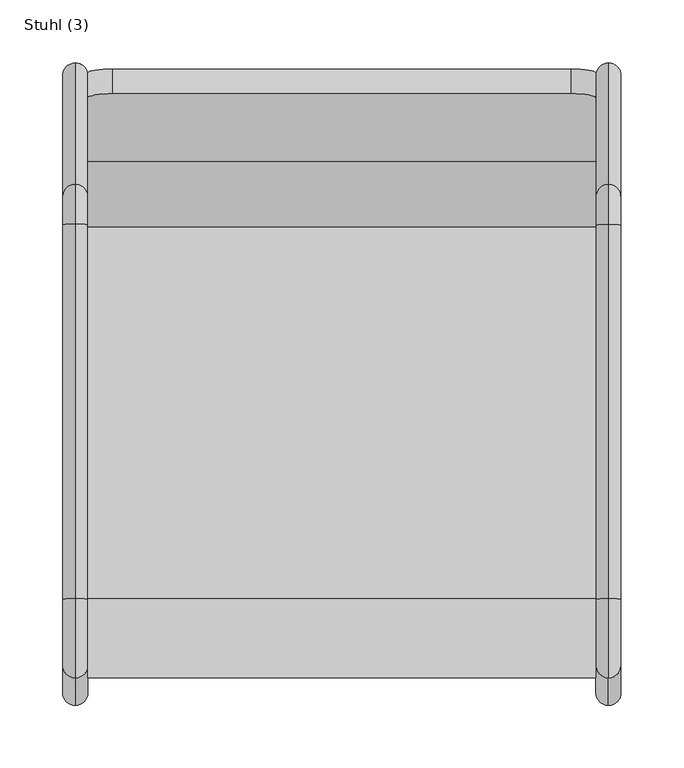
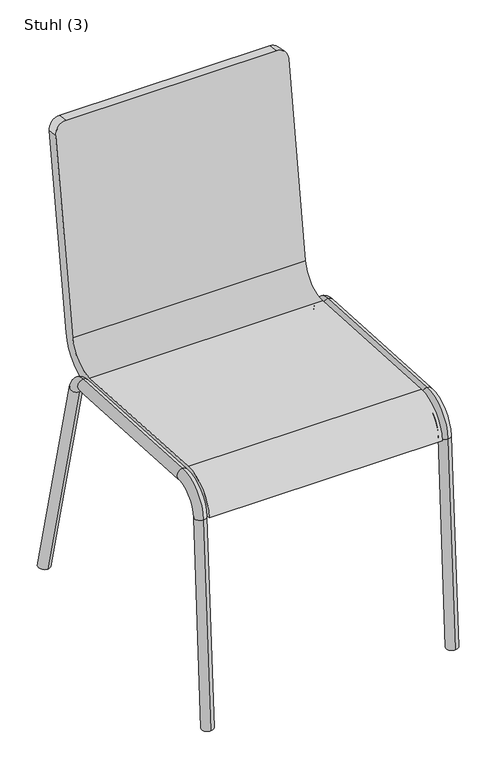
"""IFC4 building model written with IfcOpenShell, lengths in millimetres: furniture geometry, Stuhl (3) : Sessel."""

from ifc_helpers import new_model, si_unit, point, frame, origin, place, context, project, spatial, polyline, circle_curve, ellipse_curve, trimmed, source, transform, mapped, element, save
from ifc_brep_helpers import plane_surface, cylinder_surface, revolved_surface, advanced_brep


def stuhl_3_dbe21b2d(model_context):
    return source(origin(), model_context, "Body", "AdvancedBrep", [
        advanced_brep(
        [(-139.5255992, 4.9530016, 0.0), (-139.5255992, 25.5652742, 0.0), (-129.5255992, -476.7023393, 0.0), (-149.5255992, -476.7023393, 0.0), (-139.5255992, -466.6854234, 0.0), (-139.5255992, -90.5686349, 383.1163586), (-139.5255992, -71.1627204, 387.9547965), (-139.5255992, -104.2517001, 394.4621992), (-139.5255992, -103.0898724, 414.4284246), (-139.5255992, -402.6537429, 411.8261096), (-139.5255992, -401.4919152, 431.792335), (-139.5255992, -444.909849, 374.2173141), (-139.5255992, -464.8760744, 375.3791418), (-139.5255992, -486.685452, 0.5809138)],
        [
            (0, 1, ellipse_curve(frame((-139.5255992, 15.2591379, 0.0), z_axis=(0.0, 0.0, -1.0), x_axis=(0.0, 1.0, 0.0)), 10.3061363, 10.0)),
            (1, 0, ellipse_curve(frame((-139.5255992, 15.2591379, 0.0), z_axis=(0.0, 0.0, -1.0), x_axis=(0.0, 1.0, 0.0)), 10.3061363, 10.0)),
            (2, 3),
            (3, 4, ellipse_curve(frame((-139.5255992, -476.7023393, 0.0), z_axis=(0.0, 0.0, -1.0), x_axis=(0.0, 1.0, 0.0)), 10.0169159, 10.0)),
            (4, 2, ellipse_curve(frame((-139.5255992, -476.7023393, 0.0), z_axis=(0.0, 0.0, -1.0), x_axis=(0.0, 1.0, 0.0)), 10.0169159, 10.0)),
            (5, 6, circle_curve(frame((-139.5255992, -80.8656776, 385.5355776), z_axis=(0.0, 0.24192189559966623, -0.9702957262759968), x_axis=(0.0, 0.9702957262759968, 0.24192189559966623)), 10.0)),
            (6, 1),
            (0, 5),
            (6, 5, circle_curve(frame((-139.5255992, -80.8656776, 385.5355776), z_axis=(0.0, 0.24192189559966623, -0.9702957262759968), x_axis=(0.0, 0.9702957262759968, 0.24192189559966623)), 10.0)),
            (5, 7, circle_curve(frame((-139.5255992, -105.1230708, 379.4875302), z_axis=(1.0, 0.0, 0.0), x_axis=(0.0, 0.9702957262759969, 0.2419218955996659)), 15.0)),
            (7, 8, circle_curve(frame((-139.5255992, -103.6707862, 404.4453119), z_axis=(0.0, 0.998311269703977, -0.058091383027376764), x_axis=(0.0, 0.058091383027376764, 0.998311269703977)), 10.0)),
            (8, 6, circle_curve(frame((-139.5255992, -105.1230708, 379.4875302), z_axis=(-1.0, 0.0, 0.0), x_axis=(0.0, 0.9702957262759969, 0.2419218955996659)), 35.0)),
            (8, 7, circle_curve(frame((-139.5255992, -103.6707862, 404.4453119), z_axis=(0.0, 0.9983112697039765, -0.05809138302738498), x_axis=(0.0, 0.05809138302738498, 0.9983112697039765)), 10.0)),
            (7, 9),
            (9, 10, circle_curve(frame((-139.5255992, -402.0728291, 421.8092223), z_axis=(0.0, 0.9983112697039764, -0.058091383027386895), x_axis=(0.0, 0.058091383027386895, 0.9983112697039764)), 10.0)),
            (10, 8),
            (10, 9, circle_curve(frame((-139.5255992, -402.0728291, 421.8092223), z_axis=(0.0, 0.9983112697039764, -0.058091383027386895), x_axis=(0.0, 0.058091383027386895, 0.9983112697039764)), 10.0)),
            (9, 11, circle_curve(frame((-139.5255992, -404.9773982, 371.8936588), z_axis=(1.0, 0.0, 0.0), x_axis=(0.0, 0.05809138302738633, 0.9983112697039764)), 40.0)),
            (11, 12, circle_curve(frame((-139.5255992, -454.8929617, 374.7982279), z_axis=(0.0, 0.058091383027391474, 0.9983112697039761), x_axis=(0.0, -0.9983112697039761, 0.058091383027391474)), 10.0)),
            (12, 10, circle_curve(frame((-139.5255992, -404.9773982, 371.8936588), z_axis=(-1.0, 0.0, 0.0), x_axis=(0.0, 0.05809138302738633, 0.9983112697039764)), 60.0)),
            (12, 11, circle_curve(frame((-139.5255992, -454.8929617, 374.7982279), z_axis=(0.0, 0.05809138302739081, 0.9983112697039762), x_axis=(0.0, -0.9983112697039762, 0.05809138302739081)), 10.0)),
            (2, 13, circle_curve(frame((-139.5255992, -476.7023393, 0.0), z_axis=(0.0, -0.058091383027392335, -0.9983112697039761), x_axis=(0.0, -0.9983112697039761, 0.058091383027392335)), 10.0)),
            (13, 3, circle_curve(frame((-139.5255992, -476.7023393, 0.0), z_axis=(0.0, -0.058091383027392335, -0.9983112697039761), x_axis=(0.0, -0.9983112697039761, 0.058091383027392335)), 10.0)),
            (11, 4),
            (13, 12),
        ],
        [
            plane_surface(frame((-102.1053, 50.7055201, 0.0), z_axis=(0.0, 0.0, -1.0), x_axis=(-1.0, 0.0, 0.0))),
            cylinder_surface(frame((-139.5255992, 17.8692882, -10.4687411), z_axis=(0.0, 0.24192189559966623, -0.9702957262759968), x_axis=(0.0, 0.9702957262759968, 0.24192189559966623)), 10.0),
            revolved_surface(trimmed(ellipse_curve(frame((-139.5255992, -80.8656776, 385.5355776), z_axis=(0.0, 0.2419218955996659, -0.9702957262759969), x_axis=(0.0, 0.9702957262759969, 0.2419218955996659)), 10.0, 10.0), [point((-139.5255992, -90.5686349, 383.1163586))], [point((-139.5255992, -71.1627204, 387.9547965))], True, "CARTESIAN"), (-159.5255992, -105.1230708, 379.4875302), (1.0, 0.0, 0.0)),
            revolved_surface(trimmed(ellipse_curve(frame((-139.5255992, -80.8656776, 385.5355776), z_axis=(0.0, 0.2419218955996659, -0.9702957262759969), x_axis=(0.0, 0.9702957262759969, 0.2419218955996659)), 10.0, 10.0), [point((-139.5255992, -71.1627204, 387.9547965))], [point((-139.5255992, -90.5686349, 383.1163586))], True, "CARTESIAN"), (-159.5255992, -105.1230708, 379.4875302), (1.0, 0.0, 0.0)),
            cylinder_surface(frame((-139.5255992, -103.6707862, 404.4453119), z_axis=(0.0, 0.9983112697039764, -0.058091383027386895), x_axis=(0.0, 0.058091383027386895, 0.9983112697039764)), 10.0),
            revolved_surface(trimmed(ellipse_curve(frame((-139.5255992, -402.0728291, 421.8092223), z_axis=(0.0, 0.9983112697039764, -0.05809138302738631), x_axis=(0.0, 0.05809138302738631, 0.9983112697039764)), 10.0, 10.0), [point((-139.5255992, -402.6537429, 411.8261096))], [point((-139.5255992, -401.4919152, 431.792335))], True, "CARTESIAN"), (-159.5255992, -404.9773982, 371.8936588), (1.0, 0.0, 0.0)),
            revolved_surface(trimmed(ellipse_curve(frame((-139.5255992, -402.0728291, 421.8092223), z_axis=(0.0, 0.9983112697039764, -0.05809138302738631), x_axis=(0.0, 0.05809138302738631, 0.9983112697039764)), 10.0, 10.0), [point((-139.5255992, -401.4919152, 431.792335))], [point((-139.5255992, -402.6537429, 411.8261096))], True, "CARTESIAN"), (-159.5255992, -404.9773982, 371.8936588), (1.0, 0.0, 0.0)),
            plane_surface(frame((-159.5255992, -476.7023393, 0.0), z_axis=(0.0, -0.058091383027392335, -0.9983112697039761), x_axis=(1.0, 0.0, 0.0))),
            cylinder_surface(frame((-139.5255992, -454.8929617, 374.7982279), z_axis=(0.0, 0.058091383027392335, 0.9983112697039761), x_axis=(0.0, -0.9983112697039761, 0.058091383027392335)), 10.0),
        ],
        [
            (0, [[1, 2]]),
            (0, [[3, 4, 5]]),
            (1, [[6, 7, -1, 8]]),
            (1, [[9, -8, -2, -7]]),
            (2, [[-6, 10, 11, 12]]),
            (3, [[-9, -12, 13, -10]]),
            (4, [[-11, 14, 15, 16]]),
            (4, [[-13, -16, 17, -14]]),
            (5, [[-15, 18, 19, 20]]),
            (6, [[-17, -20, 21, -18]]),
            (7, [[22, 23, -3]]),
            (8, [[-19, 24, -4, -23, 25]]),
            (8, [[-21, -25, -22, -5, -24]]),
        ],
    ),
        advanced_brep(
        [(-554.6850007, -476.7023393, 0.0), (-564.6850007, -486.685452, 0.5809138), (-574.6850007, -476.7023393, 0.0), (-564.6850007, -90.5686349, 383.1163586), (-564.6850007, -71.1627204, 387.9547965), (-564.6850007, 25.5652742, 0.0), (-564.6850007, 4.9530016, 0.0), (-564.6850007, -466.6854234, 0.0), (-564.6850007, -103.0898724, 414.4284246), (-564.6850007, -104.2517001, 394.4621992), (-564.6850007, -402.6537429, 411.8261096), (-564.6850007, -401.4919152, 431.792335), (-564.6850007, -444.909849, 374.2173141), (-564.6850007, -464.8760744, 375.3791418)],
        [
            (0, 1, circle_curve(frame((-564.6850007, -476.7023393, 0.0), z_axis=(0.0, -0.058091383027392335, -0.9983112697039761), x_axis=(0.0, -0.9983112697039761, 0.058091383027392335)), 10.0)),
            (1, 2, circle_curve(frame((-564.6850007, -476.7023393, 0.0), z_axis=(0.0, -0.058091383027392335, -0.9983112697039761), x_axis=(0.0, -0.9983112697039761, 0.058091383027392335)), 10.0)),
            (2, 0),
            (3, 4, circle_curve(frame((-564.6850007, -80.8656776, 385.5355776), z_axis=(0.0, 0.24192189559966623, -0.9702957262759968), x_axis=(0.0, 0.9702957262759968, 0.24192189559966623)), 10.0)),
            (4, 5),
            (5, 6, ellipse_curve(frame((-564.6850007, 15.2591379, 0.0), z_axis=(0.0, 0.0, 1.0), x_axis=(0.0, 1.0, 0.0)), 10.3061363, 10.0)),
            (6, 3),
            (4, 3, circle_curve(frame((-564.6850007, -80.8656776, 385.5355776), z_axis=(0.0, 0.24192189559966623, -0.9702957262759968), x_axis=(0.0, 0.9702957262759968, 0.24192189559966623)), 10.0)),
            (6, 5, ellipse_curve(frame((-564.6850007, 15.2591379, 0.0), z_axis=(0.0, 0.0, 1.0), x_axis=(0.0, 1.0, 0.0)), 10.3061363, 10.0)),
            (2, 7, ellipse_curve(frame((-564.6850007, -476.7023393, 0.0), z_axis=(0.0, 0.0, -1.0), x_axis=(0.0, 1.0, 0.0)), 10.0169159, 10.0)),
            (7, 0, ellipse_curve(frame((-564.6850007, -476.7023393, 0.0), z_axis=(0.0, 0.0, -1.0), x_axis=(0.0, 1.0, 0.0)), 10.0169159, 10.0)),
            (8, 9, circle_curve(frame((-564.6850007, -103.6707862, 404.4453119), z_axis=(0.0, -0.9983112697039764, 0.058091383027386895), x_axis=(0.0, 0.058091383027386895, 0.9983112697039764)), 10.0)),
            (9, 10),
            (10, 11, circle_curve(frame((-564.6850007, -402.0728291, 421.8092223), z_axis=(0.0, 0.9983112697039764, -0.058091383027386895), x_axis=(0.0, 0.058091383027386895, 0.9983112697039764)), 10.0)),
            (11, 8),
            (9, 8, circle_curve(frame((-564.6850007, -103.6707862, 404.4453119), z_axis=(0.0, -0.9983112697039764, 0.058091383027386895), x_axis=(0.0, 0.058091383027386895, 0.9983112697039764)), 10.0)),
            (11, 10, circle_curve(frame((-564.6850007, -402.0728291, 421.8092223), z_axis=(0.0, 0.9983112697039764, -0.058091383027386895), x_axis=(0.0, 0.058091383027386895, 0.9983112697039764)), 10.0)),
            (10, 12, circle_curve(frame((-564.6850007, -404.9773982, 371.8936588), z_axis=(1.0, 0.0, 0.0), x_axis=(0.0, 0.05809138302738633, 0.9983112697039764)), 40.0)),
            (12, 13, circle_curve(frame((-564.6850007, -454.8929617, 374.7982279), z_axis=(0.0, 0.058091383027391474, 0.9983112697039761), x_axis=(0.0, -0.9983112697039761, 0.058091383027391474)), 10.0)),
            (13, 11, circle_curve(frame((-564.6850007, -404.9773982, 371.8936588), z_axis=(-1.0, 0.0, 0.0), x_axis=(0.0, 0.05809138302738633, 0.9983112697039764)), 60.0)),
            (13, 12, circle_curve(frame((-564.6850007, -454.8929617, 374.7982279), z_axis=(0.0, 0.05809138302739081, 0.9983112697039762), x_axis=(0.0, -0.9983112697039762, 0.05809138302739081)), 10.0)),
            (12, 7),
            (1, 13),
            (3, 9, circle_curve(frame((-564.6850007, -105.1230708, 379.4875302), z_axis=(1.0, 0.0, 0.0), x_axis=(0.0, 0.9702957262759969, 0.2419218955996659)), 15.0)),
            (8, 4, circle_curve(frame((-564.6850007, -105.1230708, 379.4875302), z_axis=(-1.0, 0.0, 0.0), x_axis=(0.0, 0.9702957262759969, 0.2419218955996659)), 35.0)),
        ],
        [
            plane_surface(frame((-544.6850007, -476.7023393, 0.0), z_axis=(0.0, -0.058091383027392335, -0.9983112697039761), x_axis=(-1.0, 0.0, 0.0))),
            cylinder_surface(frame((-564.6850007, 17.8692882, -10.4687411), z_axis=(0.0, 0.24192189559966623, -0.9702957262759968), x_axis=(0.0, 0.9702957262759968, 0.24192189559966623)), 10.0),
            plane_surface(frame((-102.1053, 50.7055201, 0.0), z_axis=(0.0, 0.0, -1.0), x_axis=(-1.0, 0.0, 0.0))),
            cylinder_surface(frame((-564.6850007, -103.6707862, 404.4453119), z_axis=(0.0, 0.9983112697039764, -0.058091383027386895), x_axis=(0.0, 0.058091383027386895, 0.9983112697039764)), 10.0),
            revolved_surface(trimmed(ellipse_curve(frame((-564.6850007, -402.0728291, 421.8092223), z_axis=(0.0, 0.9983112697039764, -0.05809138302738631), x_axis=(0.0, 0.05809138302738631, 0.9983112697039764)), 10.0, 10.0), [point((-564.6850007, -402.6537429, 411.8261096))], [point((-564.6850007, -401.4919152, 431.792335))], True, "CARTESIAN"), (-544.6850007, -404.9773982, 371.8936588), (1.0, 0.0, 0.0)),
            revolved_surface(trimmed(ellipse_curve(frame((-564.6850007, -402.0728291, 421.8092223), z_axis=(0.0, 0.9983112697039764, -0.05809138302738631), x_axis=(0.0, 0.05809138302738631, 0.9983112697039764)), 10.0, 10.0), [point((-564.6850007, -401.4919152, 431.792335))], [point((-564.6850007, -402.6537429, 411.8261096))], True, "CARTESIAN"), (-544.6850007, -404.9773982, 371.8936588), (1.0, 0.0, 0.0)),
            cylinder_surface(frame((-564.6850007, -454.8929617, 374.7982279), z_axis=(0.0, 0.058091383027392335, 0.9983112697039761), x_axis=(0.0, -0.9983112697039761, 0.058091383027392335)), 10.0),
            revolved_surface(trimmed(ellipse_curve(frame((-564.6850007, -80.8656776, 385.5355776), z_axis=(0.0, 0.2419218955996659, -0.9702957262759969), x_axis=(0.0, 0.9702957262759969, 0.2419218955996659)), 10.0, 10.0), [point((-564.6850007, -90.5686349, 383.1163586))], [point((-564.6850007, -71.1627204, 387.9547965))], True, "CARTESIAN"), (-544.6850007, -105.1230708, 379.4875302), (1.0, 0.0, 0.0)),
            revolved_surface(trimmed(ellipse_curve(frame((-564.6850007, -80.8656776, 385.5355776), z_axis=(0.0, 0.2419218955996659, -0.9702957262759969), x_axis=(0.0, 0.9702957262759969, 0.2419218955996659)), 10.0, 10.0), [point((-564.6850007, -71.1627204, 387.9547965))], [point((-564.6850007, -90.5686349, 383.1163586))], True, "CARTESIAN"), (-544.6850007, -105.1230708, 379.4875302), (1.0, 0.0, 0.0)),
        ],
        [
            (0, [[1, 2, 3]]),
            (1, [[4, 5, 6, 7]]),
            (1, [[8, -7, 9, -5]]),
            (2, [[-3, 10, 11]]),
            (2, [[-6, -9]]),
            (3, [[12, 13, 14, 15]]),
            (3, [[16, -15, 17, -13]]),
            (4, [[-14, 18, 19, 20]]),
            (5, [[-17, -20, 21, -18]]),
            (6, [[-19, 22, -10, -2, 23]]),
            (6, [[-21, -23, -1, -11, -22]]),
            (7, [[-4, 24, -12, 25]]),
            (8, [[-8, -25, -16, -24]]),
        ],
    ),
        advanced_brep(
        [(-149.6053, -105.450673, 414.5657988), (-149.6053, -401.4919152, 431.792335), (-149.6053, -464.8760744, 375.3791418), (-149.6053, -444.909849, 374.2173141), (-149.6053, -402.6537429, 411.8261096), (-149.6053, -106.6125007, 394.5995734), (-149.6053, -33.3149934, 454.1347035), (-149.6053, 17.5412109, 794.4215124), (-149.6053, -2.2391064, 797.3777006), (-149.6053, -53.0953107, 457.0908917), (-554.6053, -105.450673, 414.5657988), (-554.6053, -53.0953107, 457.0908917), (-554.6053, -2.2391064, 797.3777006), (-554.6053, 17.5412109, 794.4215124), (-554.6053, -33.3149934, 454.1347035), (-554.6053, -106.6125007, 394.5995734), (-554.6053, -402.6537429, 411.8261096), (-554.6053, -444.909849, 374.2173141), (-554.6053, -464.8760744, 375.3791418), (-554.6053, -401.4919152, 431.792335), (-534.6053, 20.4973991, 814.2018297), (-169.6053, 20.4973991, 814.2018297), (-534.6053, 0.7170819, 817.1580179), (-169.6053, 0.7170819, 817.1580179)],
        [
            (0, 1),
            (1, 2, circle_curve(frame((-149.6053, -404.9773982, 371.8936588), z_axis=(1.0, 0.0, 0.0), x_axis=(0.0, 1.0, 0.0)), 60.0)),
            (2, 3),
            (3, 4, circle_curve(frame((-149.6053, -404.9773982, 371.8936588), z_axis=(-1.0, 0.0, 0.0), x_axis=(0.0, 1.0, 0.0)), 40.0)),
            (4, 5),
            (5, 6, circle_curve(frame((-149.6053, -102.5461039, 464.4813623), z_axis=(1.0, 0.0, 0.0), x_axis=(0.0, 1.0, 0.0)), 70.0)),
            (6, 7),
            (7, 8),
            (8, 9),
            (9, 0, circle_curve(frame((-149.6053, -102.5461039, 464.4813623), z_axis=(-1.0, 0.0, 0.0), x_axis=(0.0, 1.0, 0.0)), 50.0)),
            (10, 11, circle_curve(frame((-554.6053, -102.5461039, 464.4813623), z_axis=(1.0, 0.0, 0.0), x_axis=(0.0, 1.0, 0.0)), 50.0)),
            (11, 12),
            (12, 13),
            (13, 14),
            (14, 15, circle_curve(frame((-554.6053, -102.5461039, 464.4813623), z_axis=(-1.0, 0.0, 0.0), x_axis=(0.0, 1.0, 0.0)), 70.0)),
            (15, 16),
            (16, 17, circle_curve(frame((-554.6053, -404.9773982, 371.8936588), z_axis=(1.0, 0.0, 0.0), x_axis=(0.0, 1.0, 0.0)), 40.0)),
            (17, 18),
            (18, 19, circle_curve(frame((-554.6053, -404.9773982, 371.8936588), z_axis=(-1.0, 0.0, 0.0), x_axis=(0.0, 1.0, 0.0)), 60.0)),
            (19, 10),
            (0, 10),
            (19, 1),
            (18, 2),
            (17, 3),
            (16, 4),
            (15, 5),
            (14, 6),
            (13, 20, circle_curve(frame((-534.6053, 17.5412109, 794.4215124), z_axis=(0.0, 0.9890158633619166, -0.14780941112961252), x_axis=(1.0, 0.0, 0.0)), 20.0)),
            (20, 21),
            (21, 7, circle_curve(frame((-169.6053, 17.5412109, 794.4215124), z_axis=(0.0, 0.9890158633619166, -0.14780941112961252), x_axis=(-1.0, 0.0, 0.0)), 20.0)),
            (20, 22),
            (22, 23),
            (23, 21),
            (11, 9),
            (8, 23, circle_curve(frame((-169.6053, -2.2391064, 797.3777006), z_axis=(0.0, -0.9890158633619166, 0.14780941112961252), x_axis=(-1.0, 0.0, 0.0)), 20.0)),
            (22, 12, circle_curve(frame((-534.6053, -2.2391064, 797.3777006), z_axis=(0.0, -0.9890158633619166, 0.14780941112961252), x_axis=(1.0, 0.0, 0.0)), 20.0)),
        ],
        [
            plane_surface(frame((-149.6053, -399.2468499, 431.6616954), z_axis=(1.0000000000000002, 0.0, 0.0), x_axis=(0.0, -0.9983112697039764, 0.05809138302738736))),
            plane_surface(frame((-554.6053, -399.2468499, 431.6616954), z_axis=(-1.0000000000000002, 0.0, 0.0), x_axis=(0.0, 0.9983112697039764, -0.05809138302738736))),
            plane_surface(frame((-149.6053, -105.450673, 414.5657988), z_axis=(0.0, 0.05809138302738736, 0.9983112697039764), x_axis=(-1.0, 0.0, 0.0))),
            cylinder_surface(frame((-554.6053, -404.9773982, 371.8936588), z_axis=(1.0, 0.0, 0.0), x_axis=(0.0, 1.0, 0.0)), 60.0),
            plane_surface(frame((-149.6053, -464.8760744, 375.3791418), z_axis=(0.0, -0.058091383027390926, -0.9983112697039762), x_axis=(-1.0, 0.0, 0.0))),
            revolved_surface(polyline([(-554.6053, -364.9773982, 371.8936588), (-149.6053, -364.9773982, 371.8936588)]), (-554.6053, -404.9773982, 371.8936588), (-1.0, 0.0, 0.0)),
            plane_surface(frame((-149.6053, -402.6537429, 411.8261096), z_axis=(0.0, -0.05809138302738756, -0.9983112697039763), x_axis=(-1.0, 0.0, 0.0))),
            cylinder_surface(frame((-554.6053, -102.5461039, 464.4813623), z_axis=(1.0, 0.0, 0.0), x_axis=(0.0, 1.0, 0.0)), 70.0),
            plane_surface(frame((-149.6053, -33.3149934, 454.1347035), z_axis=(0.0, 0.9890158633619166, -0.1478094111296125), x_axis=(-1.0, 0.0, 0.0))),
            plane_surface(frame((-149.6053, 20.4973991, 814.2018297), z_axis=(0.0, 0.14780941112961524, 0.9890158633619162), x_axis=(-1.0, 0.0, 0.0))),
            plane_surface(frame((-149.6053, 0.7170819, 817.1580179), z_axis=(0.0, -0.9890158633619166, 0.14780941112961254), x_axis=(-1.0, 0.0, 0.0))),
            revolved_surface(polyline([(-554.6053, -52.546103900000006, 464.4813623), (-149.6053, -52.546103900000006, 464.4813623)]), (-554.6053, -102.5461039, 464.4813623), (-1.0, 0.0, 0.0)),
            cylinder_surface(frame((-534.6053, -2.2391064, 797.3777006), z_axis=(0.0, -0.9890158633619166, 0.14780941112961252), x_axis=(1.0, 0.0, 0.0)), 20.0),
            cylinder_surface(frame((-169.6053, -2.2391064, 797.3777006), z_axis=(0.0, -0.9890158633619166, 0.14780941112961252), x_axis=(-1.0, 0.0, 0.0)), 20.0),
        ],
        [
            (0, [[1, 2, 3, 4, 5, 6, 7, 8, 9, 10]]),
            (1, [[11, 12, 13, 14, 15, 16, 17, 18, 19, 20]]),
            (2, [[-1, 21, -20, 22]]),
            (3, [[-2, -22, -19, 23]]),
            (4, [[-3, -23, -18, 24]]),
            (5, [[-4, -24, -17, 25]]),
            (6, [[-5, -25, -16, 26]]),
            (7, [[-6, -26, -15, 27]]),
            (8, [[-27, -14, 28, 29, 30, -7]]),
            (9, [[-29, 31, 32, 33]]),
            (10, [[34, -9, 35, -32, 36, -12]]),
            (11, [[-10, -34, -11, -21]]),
            (12, [[-13, -36, -31, -28]]),
            (13, [[-8, -30, -33, -35]]),
        ],
    ),
    ])


if __name__ == "__main__":
    model = new_model("IFC4")
    model_context = context("Model", 3, world=origin())
    ifc_project = project(units=[si_unit("LENGTHUNIT", "METRE", prefix="MILLI")], contexts=[model_context])
    site = spatial("IfcSite", under=ifc_project)
    building = spatial("IfcBuilding", under=site)
    placement = place(None, origin())
    stuhl_3_shape = stuhl_3_dbe21b2d(model_context)
    element("IfcFurniture", 1, ObjectType="Stuhl (3) : Sessel", at=placement, inside=building, context=model_context, shape_type="MappedRepresentation", body=[
        mapped(stuhl_3_shape, transform((0.0, 0.0, 0.0), x_axis=(1.0, 0.0, 0.0), y_axis=(0.0, 1.0, 0.0), z_axis=(0.0, 0.0, 1.0))),
    ])
    save(model, "model.ifc")

# Revit data of these elements
# Type "Stuhl (3) : Sessel"
#   Im Vordergrund zeichnen [instance default] = yes
#   Stuhllehne = Kunststoff - Grau
#   Füsse = Metall - Aluminium
#   Model = ""
#   Manufacturer = ""
#   Description = (empty or 0)
# Element 1 (IfcFurniture, "Stuhl (3) : Sessel")
#   Materials on its faces: "Metall - Aluminium", "Kunststoff - Grau"
# Materials
#   "Kunststoff - Grau": class "Kunststoff", colour RGB 127 127 127, transparency 0, Cost = 0
#   "Metall - Aluminium": class "Metall", colour RGB 247 247 247, transparency 0, Description = "Aluminium 6061", Cost = 0
